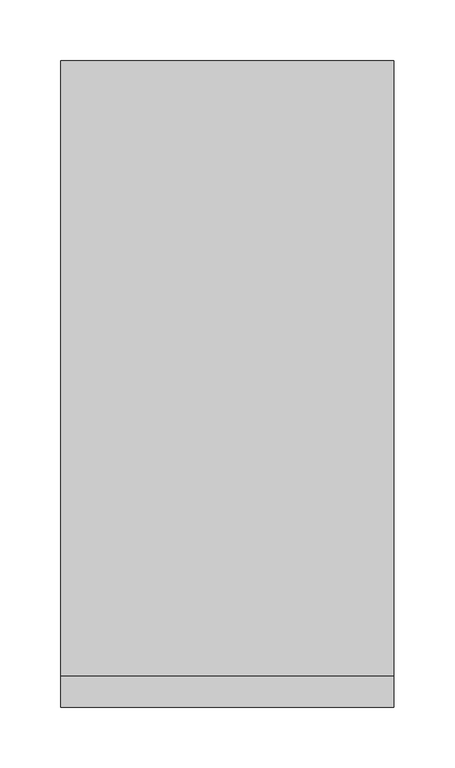
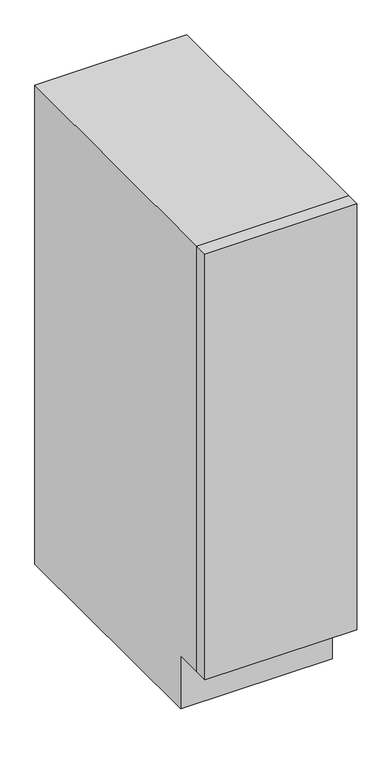
"""IFC4 building model written with IfcOpenShell, lengths in millimetres: furniture geometry, OD_CW_Base Cabinet : OD_CW_Base Cabinet."""

from ifc_helpers import new_model, si_unit, frame, origin, place, context, project, spatial, polyline, outline, extrude, source, transform, mapped, element, save


def furniture_b87d32b9(model_context):
    return source(origin(), model_context, "Body", "SweptSolid", [
        extrude(outline(polyline([(18.7377049, 103.0908776), (292.9657997, 103.0908776), (292.9657997, 77.6908776), (18.7377049, 77.6908776), (18.7377049, 103.0908776)])), frame((0.0, 0.0, 101.6), z_axis=(0.0, 0.0, 1.0), x_axis=(1.0, 0.0, 0.0)), (0.0, 0.0, 1.0), 812.8),
        extrude(outline(polyline([(103.0908776, 914.4), (609.6, 914.4), (609.6, 0.0), (153.8908776, 0.0), (153.8908776, 101.6), (103.0908776, 101.6), (103.0908776, 914.4)])), frame((18.7377049, 0.0, 0.0), z_axis=(1.0, 0.0, 0.0), x_axis=(0.0, 1.0, 0.0)), (0.0, 0.0, 1.0), 274.2280948),
    ])


if __name__ == "__main__":
    model = new_model("IFC4")
    model_context = context("Model", 3, world=origin())
    ifc_project = project(units=[si_unit("LENGTHUNIT", "METRE", prefix="MILLI")], contexts=[model_context])
    site = spatial("IfcSite", under=ifc_project)
    building = spatial("IfcBuilding", under=site)
    placement = place(None, origin())
    furniture_shape = furniture_b87d32b9(model_context)
    element("IfcFurniture", 1, ObjectType="OD_CW_Base Cabinet : OD_CW_Base Cabinet", at=placement, inside=building, context=model_context, shape_type="MappedRepresentation", body=[
        mapped(furniture_shape, transform((0.0, 0.0, 0.0), x_axis=(1.0, 0.0, 0.0), y_axis=(0.0, 1.0, 0.0), z_axis=(0.0, 0.0, 1.0))),
    ])
    save(model, "model.ifc")

# Revit data of these elements
# Type "OD_CW_Base Cabinet : OD_CW_Base Cabinet"
#   OD_CW_Width [instance default] = 2' - 10"
#   OD_CW_Length [instance default] = 8' - 0"
#   OD_CW_Height [instance default] = 2' - 3"
#   Depth = 2' - 0"
#   Height = 3' - 0"
#   Width = 4' - 0"
#   OD_CW_Material_Front Panel [instance default] = none
#   OD_CW_Material_Body [instance default] = none
# Element 1 (IfcFurniture, "OD_CW_Base Cabinet : OD_CW_Base Cabinet")
#   OD_CW_Width = 1' - 8.9413"
#   OD_CW_Length = 0' - 10.79638"
#   OD_CW_Height = 3' - 0"
#   OD_CW_Material_Body = TRASH
#   Materials on its faces: "TRASH", "CASEWORK"
# Materials
#   "TRASH": class "Generic", colour RGB 187 187 187, transparency 0, Cost = 0
#   "CASEWORK": class "Generic", colour RGB 181 181 181, transparency 0, Cost = 0
